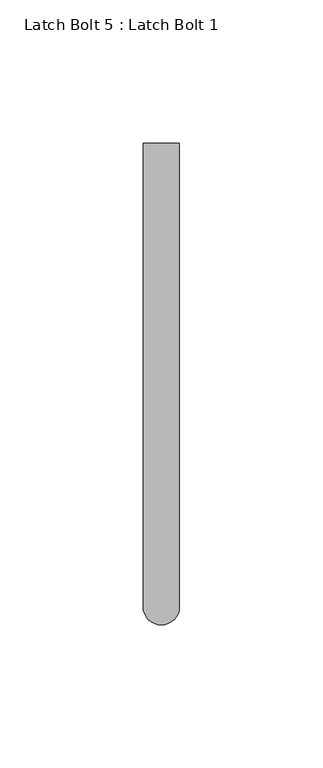
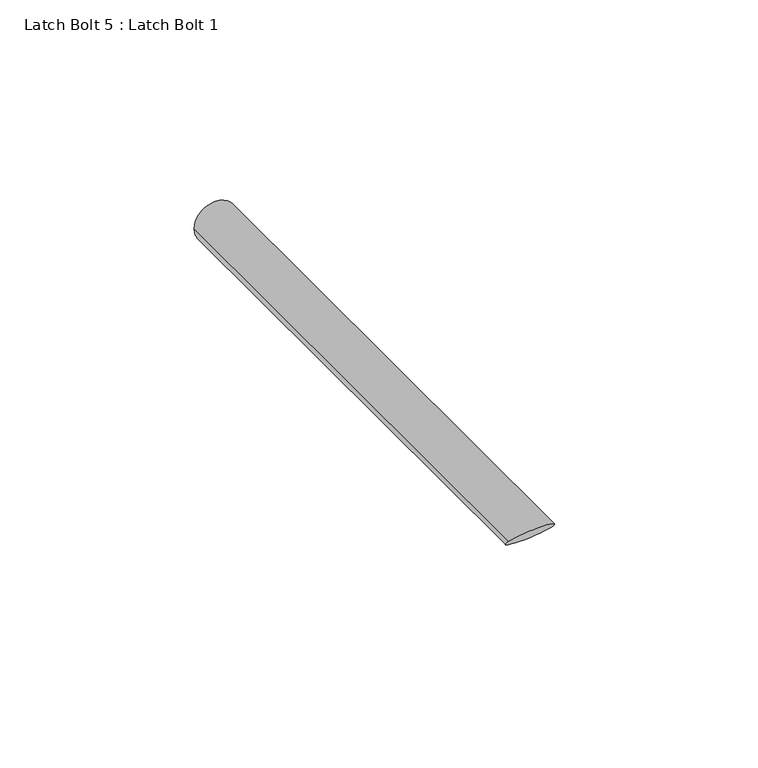
"""IFC4 building model written with IfcOpenShell, lengths in millimetres: proxy geometry, Latch Bolt 5 : Latch Bolt 1."""

from ifc_helpers import new_model, si_unit, frame, origin, place, context, project, spatial, circle_curve, ellipse_curve, source, transform, mapped, element, save
from ifc_brep_helpers import plane_surface, cylinder_surface, advanced_brep


def latch_bolt_5_latch_bolt_1_cfdedea9(model_context):
    return source(origin(), model_context, "Body", "AdvancedBrep", [
        advanced_brep(
        [(587306.3685739, -535131.7163841, 1066.8), (587319.0685739, -535131.7163841, 1066.8), (587306.3685739, -535293.6413841, 1066.8), (587312.7185739, -535299.9913841, 1073.15), (587319.0685739, -535293.6413841, 1066.8)],
        [
            (0, 1, circle_curve(frame((587312.7185739, -535131.7163841, 1066.8), z_axis=(0.0, 1.0, 0.0), x_axis=(1.0, 0.0, 0.0)), 6.35)),
            (1, 0, circle_curve(frame((587312.7185739, -535131.7163841, 1066.8), z_axis=(0.0, 1.0, 0.0), x_axis=(1.0, 0.0, 0.0)), 6.35)),
            (0, 2),
            (2, 3, ellipse_curve(frame((587312.7185739, -535293.6413841, 1066.8), z_axis=(0.0, 0.7071067811870104, 0.7071067811860847), x_axis=(0.0, 0.7071067811860846, -0.7071067811870104)), 8.9802561, 6.35)),
            (3, 4, ellipse_curve(frame((587312.7185739, -535293.6413841, 1066.8), z_axis=(0.0, 0.7071067811870104, 0.7071067811860847), x_axis=(0.0, 0.7071067811860846, -0.7071067811870104)), 8.9802561, 6.35)),
            (4, 1),
            (4, 2, ellipse_curve(frame((587312.7185739, -535293.6413841, 1066.8), z_axis=(0.0, 0.7071067811870104, 0.7071067811860847), x_axis=(0.0, 0.7071067811860846, -0.7071067811870104)), 8.9802561, 6.35)),
        ],
        [
            plane_surface(frame((587319.0685739, -535131.7163841, 1066.8), z_axis=(0.0, 1.0, 0.0), x_axis=(0.0, 0.0, -1.0))),
            cylinder_surface(frame((587312.7185739, -535299.9913841, 1066.8), z_axis=(0.0, 1.0, 0.0), x_axis=(1.0, 0.0, 0.0)), 6.35),
            plane_surface(frame((587338.1185739, -535284.1163841, 1057.275), z_axis=(0.0, -0.7071067811870104, -0.7071067811860847), x_axis=(-1.0, 0.0, 0.0))),
        ],
        [
            (0, [[1, 2]]),
            (1, [[-1, 3, 4, 5, 6]]),
            (1, [[-2, -6, 7, -3]]),
            (2, [[-4, -7, -5]]),
        ],
    ),
    ])


if __name__ == "__main__":
    model = new_model("IFC4")
    model_context = context("Model", 3, world=origin())
    ifc_project = project(units=[si_unit("LENGTHUNIT", "METRE", prefix="MILLI")], contexts=[model_context])
    site = spatial("IfcSite", under=ifc_project)
    building = spatial("IfcBuilding", under=site)
    placement = place(None, origin())
    latch_bolt_5_latch_bolt_1_shape = latch_bolt_5_latch_bolt_1_cfdedea9(model_context)
    element("IfcBuildingElementProxy", 1, Name="Latch Bolt 5 : Latch Bolt 1", ObjectType="Latch Bolt 5 : Latch Bolt 1", at=placement, inside=building, context=model_context, shape_type="MappedRepresentation", body=[
        mapped(latch_bolt_5_latch_bolt_1_shape, transform((0.0, 0.0, 0.0), x_axis=(1.0, 0.0, 0.0), y_axis=(0.0, 1.0, 0.0), z_axis=(0.0, 0.0, 1.0))),
    ])
    save(model, "model.ifc")

# Revit data of these elements
# Element 1 (IfcBuildingElementProxy, "Latch Bolt 5 : Latch Bolt 1")
#   Materials on its faces: "GALV. GATE LATCH"
# Materials
#   "GALV. GATE LATCH": class "Metal", colour RGB 189 187 185, transparency 0, Description = "Carbon steel", Cost = 0
